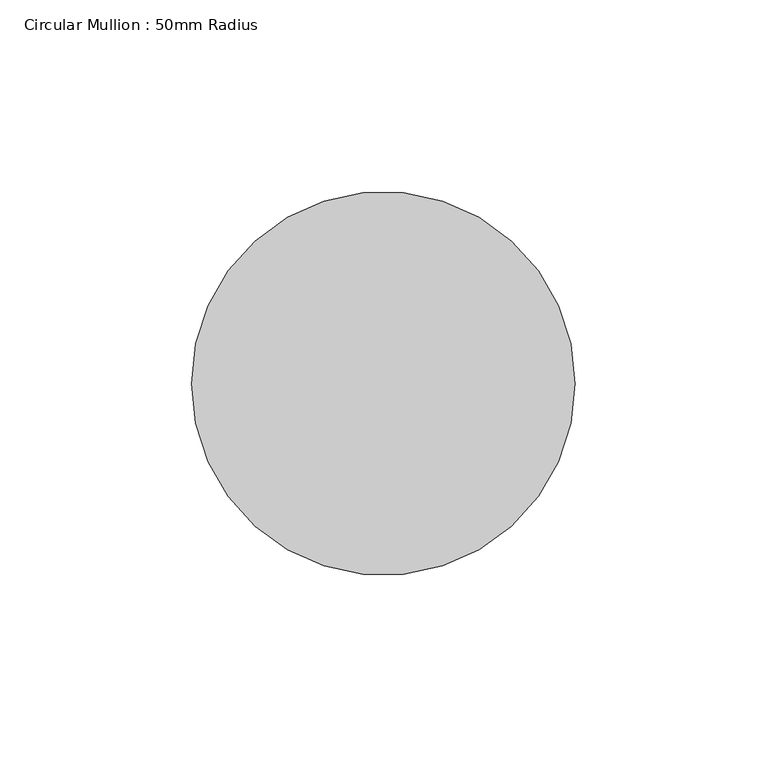
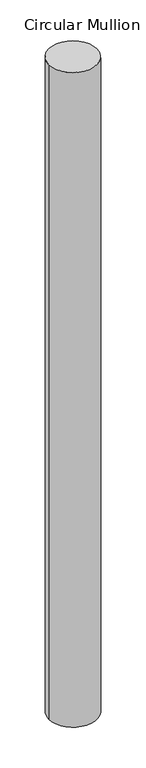
"""IFC4 building model written with IfcOpenShell, lengths in millimetres: member geometry, Circular Mullion : 50mm Radius."""

from ifc_helpers import new_model, si_unit, point, frame, origin, origin_2d, place, context, project, spatial, circle_curve, trimmed, segment, composite_curve, outline, extrude, source, transform, mapped, element, save


def circular_mullion_50mm_radius_e16bfc34(model_context):
    return source(origin(), model_context, "Body", "SweptSolid", [
        extrude(outline(composite_curve([segment(trimmed(circle_curve(origin_2d(), 50.0), [point((50.0, 0.0))], [point((-50.0, 0.0))], False, "CARTESIAN"), True, "CONTINUOUS"), segment(trimmed(circle_curve(origin_2d(), 50.0), [point((-50.0, 0.0))], [point((50.0, 0.0))], False, "CARTESIAN"), True, "CONTINUOUS")], self_intersect=False)), frame((0.0, 0.0, -1438.7947114), z_axis=(0.0, 0.0, 1.0), x_axis=(1.0, 0.0, 0.0)), (0.0, 0.0, 1.0), 1438.7947114),
    ])


if __name__ == "__main__":
    model = new_model("IFC4")
    model_context = context("Model", 3, world=origin())
    ifc_project = project(units=[si_unit("LENGTHUNIT", "METRE", prefix="MILLI")], contexts=[model_context])
    site = spatial("IfcSite", under=ifc_project)
    building = spatial("IfcBuilding", under=site)
    placement = place(None, origin())
    circular_mullion_50mm_radius_shape = circular_mullion_50mm_radius_e16bfc34(model_context)
    element("IfcMember", 1, ObjectType="Circular Mullion : 50mm Radius", at=placement, inside=building, context=model_context, shape_type="MappedRepresentation", body=[
        mapped(circular_mullion_50mm_radius_shape, transform((0.0, 0.0, 0.0), x_axis=(1.0, 0.0, 0.0), y_axis=(0.0, 1.0, 0.0), z_axis=(0.0, 0.0, 1.0))),
    ])
    save(model, "model.ifc")

# Revit data of these elements
# Type "Circular Mullion : 50mm Radius"
#   built-in parameter 1007350 = 0.164042 (stored number, unit not read)
# Element 1 (IfcMember, "Circular Mullion : 50mm Radius")
#   Materials on its faces: "Aluminium"
# Materials
#   "Aluminium": class "Metal", colour RGB 247 247 247, transparency 0, Description = "Aluminium 6061", Cost = 0
